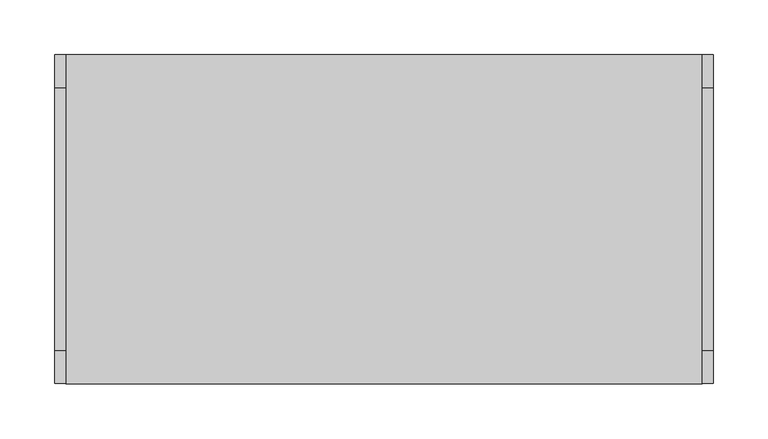
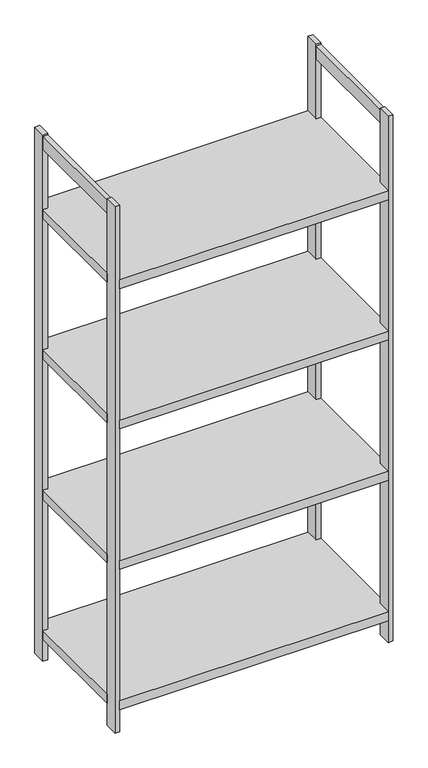
"""IFC4 building model written with IfcOpenShell, lengths in millimetres: furniture geometry, GEL-Shelf-一般オフィス棚 : GEL-Shelf-一般オフィス棚."""

from ifc_helpers import new_model, si_unit, frame, origin, origin_with_axes, place, context, project, spatial, polyline, outline, extrude, source, transform, mapped, element, save


def furniture_81dc58f3(model_context):
    return source(origin(), model_context, "Body", "SweptSolid", [
        extrude(outline(polyline([(300.0, -120.0), (290.0, -120.0), (290.0, -150.0), (-290.0, -150.0), (-290.0, -120.0), (-300.0, -120.0), (-300.0, 120.0), (-290.0, 120.0), (-290.0, 150.0), (290.0, 150.0), (290.0, 120.0), (300.0, 120.0), (300.0, -120.0)])), frame((0.0, 0.0, 50.0), z_axis=(0.0, 0.0, 1.0), x_axis=(1.0, 0.0, 0.0)), (0.0, 0.0, 1.0), 20.0),
        extrude(outline(polyline([(300.0, -120.0), (290.0, -120.0), (290.0, -150.0), (-290.0, -150.0), (-290.0, -120.0), (-300.0, -120.0), (-300.0, 120.0), (-290.0, 120.0), (-290.0, 150.0), (290.0, 150.0), (290.0, 120.0), (300.0, 120.0), (300.0, -120.0)])), frame((0.0, 0.0, 370.0), z_axis=(0.0, 0.0, 1.0), x_axis=(1.0, 0.0, 0.0)), (0.0, 0.0, 1.0), 20.0),
        extrude(outline(polyline([(300.0, -120.0), (290.0, -120.0), (290.0, -150.0), (-290.0, -150.0), (-290.0, -120.0), (-300.0, -120.0), (-300.0, 120.0), (-290.0, 120.0), (-290.0, 150.0), (290.0, 150.0), (290.0, 120.0), (300.0, 120.0), (300.0, -120.0)])), frame((0.0, 0.0, 690.0), z_axis=(0.0, 0.0, 1.0), x_axis=(1.0, 0.0, 0.0)), (0.0, 0.0, 1.0), 20.0),
        extrude(outline(polyline([(300.0, -120.0), (290.0, -120.0), (290.0, -150.0), (-290.0, -150.0), (-290.0, -120.0), (-300.0, -120.0), (-300.0, 120.0), (-290.0, 120.0), (-290.0, 150.0), (290.0, 150.0), (290.0, 120.0), (300.0, 120.0), (300.0, -120.0)])), frame((0.0, 0.0, 1010.0), z_axis=(0.0, 0.0, 1.0), x_axis=(1.0, 0.0, 0.0)), (0.0, 0.0, 1.0), 20.0),
        extrude(outline(polyline([(300.0, -150.0), (290.0, -150.0), (290.0, -120.0), (300.0, -120.0), (300.0, -150.0)])), origin_with_axes(), (0.0, 0.0, 1.0), 1200.0),
        extrude(outline(polyline([(300.0, 120.0), (290.0, 120.0), (290.0, 150.0), (300.0, 150.0), (300.0, 120.0)])), origin_with_axes(), (0.0, 0.0, 1.0), 1200.0),
        extrude(outline(polyline([(-290.0, 120.0), (-300.0, 120.0), (-300.0, 150.0), (-290.0, 150.0), (-290.0, 120.0)])), origin_with_axes(), (0.0, 0.0, 1.0), 1200.0),
        extrude(outline(polyline([(-290.0, -150.0), (-300.0, -150.0), (-300.0, -120.0), (-290.0, -120.0), (-290.0, -150.0)])), origin_with_axes(), (0.0, 0.0, 1.0), 1200.0),
        extrude(outline(polyline([(-290.0, -120.0), (-300.0, -120.0), (-300.0, 120.0), (-290.0, 120.0), (-290.0, -120.0)])), frame((0.0, 0.0, 1167.0), z_axis=(0.0, 0.0, 1.0), x_axis=(1.0, 0.0, 0.0)), (0.0, 0.0, 1.0), 30.0),
        extrude(outline(polyline([(300.0, -120.0), (290.0, -120.0), (290.0, 120.0), (300.0, 120.0), (300.0, -120.0)])), frame((0.0, 0.0, 1167.0), z_axis=(0.0, 0.0, 1.0), x_axis=(1.0, 0.0, 0.0)), (0.0, 0.0, 1.0), 30.0),
    ])


if __name__ == "__main__":
    model = new_model("IFC4")
    model_context = context("Model", 3, world=origin())
    ifc_project = project(units=[si_unit("LENGTHUNIT", "METRE", prefix="MILLI")], contexts=[model_context])
    site = spatial("IfcSite", under=ifc_project)
    building = spatial("IfcBuilding", under=site)
    placement = place(None, origin())
    furniture_shape = furniture_81dc58f3(model_context)
    element("IfcFurniture", 1, ObjectType="GEL-Shelf-一般オフィス棚 : GEL-Shelf-一般オフィス棚", at=placement, inside=building, context=model_context, shape_type="MappedRepresentation", body=[
        mapped(furniture_shape, transform((0.0, 0.0, 0.0), x_axis=(1.0, 0.0, 0.0), y_axis=(0.0, 1.0, 0.0), z_axis=(0.0, 0.0, 1.0))),
    ])
    save(model, "model.ifc")

# Revit data of these elements
# Type "GEL-Shelf-一般オフィス棚 : GEL-Shelf-一般オフィス棚"
#   GEL-Width = 600 mm
#   GEL-Height = 1200 mm
#   GEL-Depth = 300 mm
#   GEL-Material-Support = Black Opaque Plastic
#   GEL-Material-Shelf = Iroko polished
#   GEL-Material-Base = none
#   GEL-Material-Accent = none
#   Default Elevation = 0
# Element 1 (IfcFurniture, "GEL-Shelf-一般オフィス棚 : GEL-Shelf-一般オフィス棚")
#   Materials on its faces: "Iroko polished", "Black Opaque Plastic"
# Materials
#   "Black Opaque Plastic": class "一般", colour RGB 0 0 0, transparency 0, Cost = 0
#   "Iroko polished": class "一般", colour RGB 156 100 46, transparency 0, Cost = 0
